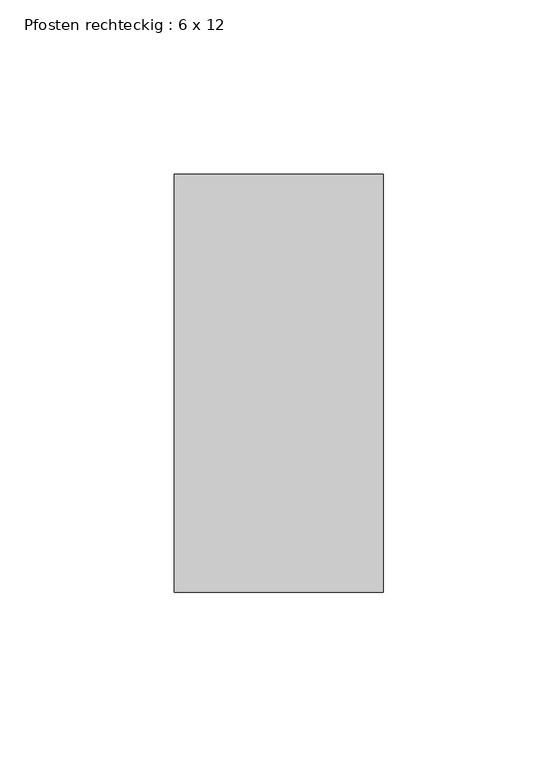
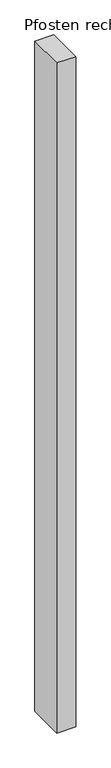
"""IFC4 building model written with IfcOpenShell, lengths in millimetres: member geometry, Pfosten rechteckig : 6 x 12."""

from ifc_helpers import new_model, si_unit, frame, origin, place, context, project, spatial, polyline, outline, extrude, source, transform, mapped, element, save


def pfosten_rechteckig_6_x_12_8f909f43(model_context):
    return source(origin(), model_context, "Body", "SweptSolid", [
        extrude(outline(polyline([(30.0, 60.0), (30.0, -60.0), (-30.0, -60.0), (-30.0, 60.0), (30.0, 60.0)])), frame((0.0, 0.0, -2250.0), z_axis=(0.0, 0.0, 1.0), x_axis=(1.0, 0.0, 0.0)), (0.0, 0.0, 1.0), 2250.0),
    ])


if __name__ == "__main__":
    model = new_model("IFC4")
    model_context = context("Model", 3, world=origin())
    ifc_project = project(units=[si_unit("LENGTHUNIT", "METRE", prefix="MILLI")], contexts=[model_context])
    site = spatial("IfcSite", under=ifc_project)
    building = spatial("IfcBuilding", under=site)
    placement = place(None, origin())
    pfosten_rechteckig_6_x_12_shape = pfosten_rechteckig_6_x_12_8f909f43(model_context)
    element("IfcMember", 1, ObjectType="Pfosten rechteckig : 6 x 12", at=placement, inside=building, context=model_context, shape_type="MappedRepresentation", body=[
        mapped(pfosten_rechteckig_6_x_12_shape, transform((0.0, 0.0, 0.0), x_axis=(1.0, 0.0, 0.0), y_axis=(0.0, 1.0, 0.0), z_axis=(0.0, 0.0, 1.0))),
    ])
    save(model, "model.ifc")

# Revit data of these elements
# Type "Pfosten rechteckig : 6 x 12"
#   built-in parameter 1007304 = 0.393701 (stored number, unit not read)
#   built-in parameter 1007301 = 0.0984252 (stored number, unit not read)
#   built-in parameter 1007300 = 0.0984252 (stored number, unit not read)
# Element 1 (IfcMember, "Pfosten rechteckig : 6 x 12")
#   Materials on its faces: "Metall - verzinkt"
# Materials
#   "Metall - verzinkt": class "Allgemeines", colour RGB 200 200 200, transparency 0, Cost = 0
